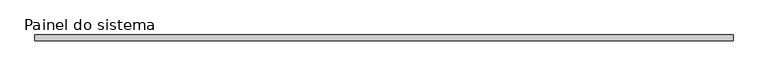
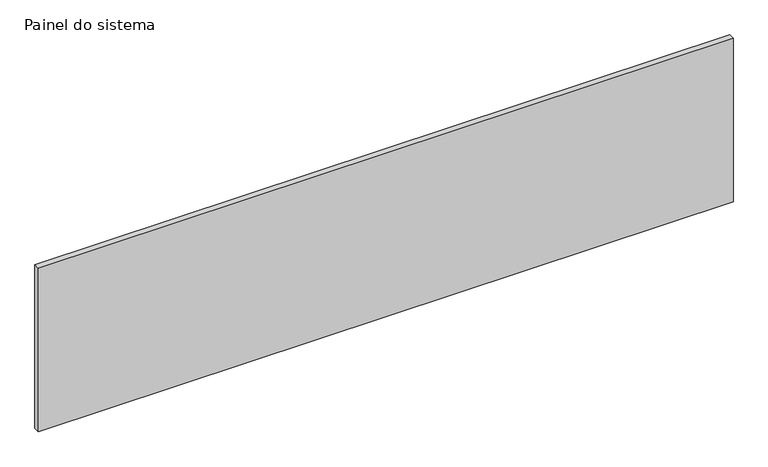
"""IFC4 building model written with IfcOpenShell, lengths in millimetres: plate geometry, Painel do sistema : Envidraçado."""

from ifc_helpers import new_model, si_unit, origin, origin_with_axes, place, context, project, spatial, polyline, outline, extrude, source, transform, mapped, element, save


def painel_do_sistema_44dfe8f0(model_context):
    return source(origin(), model_context, "Body", "SweptSolid", [
        extrude(outline(polyline([(1462.4999925, 24.5), (-1462.4999925, 24.5), (-1462.4999925, 49.5), (1462.4999925, 49.5), (1462.4999925, 24.5)])), origin_with_axes(), (0.0, 0.0, 1.0), 727.4383788),
    ])


if __name__ == "__main__":
    model = new_model("IFC4")
    model_context = context("Model", 3, world=origin())
    ifc_project = project(units=[si_unit("LENGTHUNIT", "METRE", prefix="MILLI")], contexts=[model_context])
    site = spatial("IfcSite", under=ifc_project)
    building = spatial("IfcBuilding", under=site)
    placement = place(None, origin())
    painel_do_sistema_shape = painel_do_sistema_44dfe8f0(model_context)
    element("IfcPlate", 1, ObjectType="Painel do sistema : Envidraçado", at=placement, inside=building, context=model_context, shape_type="MappedRepresentation", body=[
        mapped(painel_do_sistema_shape, transform((0.0, 0.0, 0.0), x_axis=(1.0, 0.0, 0.0), y_axis=(0.0, 1.0, 0.0), z_axis=(0.0, 0.0, 1.0))),
    ])
    save(model, "model.ifc")

# Revit data of these elements
# Type "Painel do sistema : Envidraçado"
#   Construction Type Id = "GSP4R"
#   Analytic Construction = "Vidraça única Pilkington 1/8 pol"
#   Visual Light Transmittance = 0.9
#   Solar Heat Gain Coefficient = 0.86
#   Heat Transfer Coefficient (U) = 6.7069 W/(m²·K)
# Element 1 (IfcPlate, "Painel do sistema : Envidraçado")
#   Materials on its faces: "Vidro"
# Materials
#   "Vidro": class "Vidro", colour RGB 0 128 192, transparency 0.9, Description = "Vidro de sílica", Cost = 0
